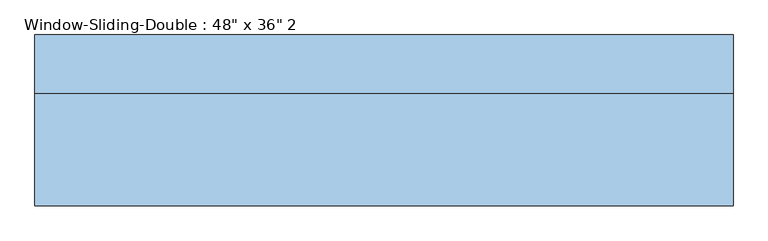
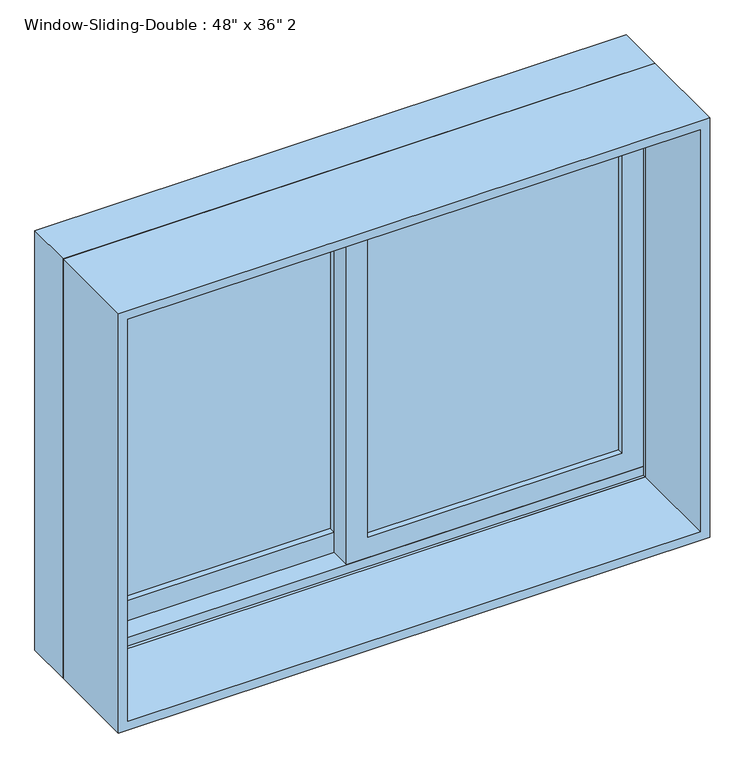
"""IFC4 building model written with IfcOpenShell, lengths in millimetres: window geometry."""

from ifc_helpers import new_model, si_unit, frame, origin, place, context, project, spatial, polyline, outline, extrude, faceted_brep, source, transform, mapped, element, save


def window_d8e423f6(model_context):
    return source(origin(), model_context, "Body", "SolidModel", [
        faceted_brep([(-609.6, 53.34, 914.4), (-609.6, 154.94, 914.4), (609.6, 154.94, 914.4), (609.6, 53.34, 914.4), (-568.6778905, 154.94, 1787.8778905), (-568.6778905, 148.59, 1787.8778905), (-568.6778905, 148.59, 933.45), (-568.6778905, 154.94, 933.45), (568.6778905, 148.59, 1787.8778905), (568.6778905, 148.59, 933.45), (590.55, 148.59, 933.45), (590.55, 148.59, 1809.75), (-590.55, 148.59, 1809.75), (-590.55, 148.59, 933.45), (-590.55, 53.34, 1809.75), (-590.55, 53.34, 933.45), (-590.55, 59.69, 933.45), (-590.55, 59.69, 952.5), (-590.55, 104.14, 952.5), (-590.55, 104.14, 933.45), (609.6, 53.34, 1828.8), (-609.6, 53.34, 1828.8), (590.55, 53.34, 1809.75), (590.55, 53.34, 933.45), (-609.6, 154.94, 1828.8), (609.6, 154.94, 1828.8), (568.6778905, 154.94, 933.45), (568.6778905, 154.94, 1787.8778905), (590.55, 104.14, 933.45), (590.55, 104.14, 952.5), (590.55, 59.69, 952.5), (590.55, 59.69, 933.45)], [[[0, 1, 2, 3]], [[4, 5, 6, 7]], [[5, 8, 9, 10, 11, 12, 13, 6]], [[12, 14, 15, 16, 17, 18, 19, 13]], [[0, 3, 20, 21], [22, 23, 15, 14]], [[24, 1, 0, 21]], [[2, 1, 24, 25], [4, 7, 26, 27]], [[5, 4, 27, 8]], [[12, 11, 22, 14]], [[21, 20, 25, 24]], [[8, 27, 26, 9]], [[22, 11, 10, 28, 29, 30, 31, 23]], [[20, 3, 2, 25]], [[26, 7, 6, 13, 19, 28, 10, 9]], [[28, 19, 18, 29]], [[29, 18, 17, 30]], [[30, 17, 16, 31]], [[15, 23, 31, 16]]]),
        extrude(outline(polyline([(1828.8, -609.6), (914.4, -609.6), (914.4, 609.6), (1828.8, 609.6), (1828.8, -609.6)]), holes=[polyline([(1809.75, 590.55), (933.45, 590.55), (933.45, -590.55), (1809.75, -590.55), (1809.75, 590.55)])]), frame((0.0, -143.51, 0.0), z_axis=(0.0, 1.0, 0.0), x_axis=(0.0, 0.0, 1.0)), (0.0, 0.0, 1.0), 196.85),
        extrude(outline(polyline([(546.1, 91.44), (546.1, 85.09), (22.225, 85.09), (22.225, 91.44), (546.1, 91.44)])), frame((0.0, 0.0, 996.95), z_axis=(0.0, 0.0, 1.0), x_axis=(1.0, 0.0, 0.0)), (0.0, 0.0, 1.0), 768.35),
        extrude(outline(polyline([(546.1, 78.74), (546.1, 72.39), (22.225, 72.39), (22.225, 78.74), (546.1, 78.74)])), frame((0.0, 0.0, 996.95), z_axis=(0.0, 0.0, 1.0), x_axis=(1.0, 0.0, 0.0)), (0.0, 0.0, 1.0), 768.35),
        extrude(outline(polyline([(-22.225, 135.89), (-22.225, 129.54), (-546.1, 129.54), (-546.1, 135.89), (-22.225, 135.89)])), frame((0.0, 0.0, 996.95), z_axis=(0.0, 0.0, 1.0), x_axis=(1.0, 0.0, 0.0)), (0.0, 0.0, 1.0), 768.35),
        extrude(outline(polyline([(-22.225, 123.19), (-22.225, 116.84), (-546.1, 116.84), (-546.1, 123.19), (-22.225, 123.19)])), frame((0.0, 0.0, 996.95), z_axis=(0.0, 0.0, 1.0), x_axis=(1.0, 0.0, 0.0)), (0.0, 0.0, 1.0), 768.35),
        extrude(outline(polyline([(933.45, -590.55), (933.45, 22.225), (1809.75, 22.225), (1809.75, -590.55), (933.45, -590.55)]), holes=[polyline([(1765.3, -22.225), (996.95, -22.225), (996.95, -546.1), (1765.3, -546.1), (1765.3, -22.225)])]), frame((0.0, 104.14, 0.0), z_axis=(0.0, 1.0, 0.0), x_axis=(0.0, 0.0, 1.0)), (0.0, 0.0, 1.0), 44.45),
        extrude(outline(polyline([(952.5, 590.55), (1809.75, 590.55), (1809.75, -22.225), (952.5, -22.225), (952.5, 590.55)]), holes=[polyline([(996.95, 22.225), (1765.3, 22.225), (1765.3, 546.1), (996.95, 546.1), (996.95, 22.225)])]), frame((0.0, 59.69, 0.0), z_axis=(0.0, 1.0, 0.0), x_axis=(0.0, 0.0, 1.0)), (0.0, 0.0, 1.0), 44.45),
    ])


if __name__ == "__main__":
    model = new_model("IFC4")
    model_context = context("Model", 3, world=origin())
    ifc_project = project(units=[si_unit("LENGTHUNIT", "METRE", prefix="MILLI")], contexts=[model_context])
    site = spatial("IfcSite", under=ifc_project)
    building = spatial("IfcBuilding", under=site)
    placement = place(None, origin())
    window_shape = window_d8e423f6(model_context)
    element("IfcWindow", 1, ObjectType="Window-Sliding-Double : 48\" x 36\" 2", at=placement, inside=building, context=model_context, shape_type="MappedRepresentation", body=[
        mapped(window_shape, transform((0.0, 0.0, 0.0), x_axis=(1.0, 0.0, 0.0), y_axis=(0.0, 1.0, 0.0), z_axis=(0.0, 0.0, 1.0))),
    ])
    save(model, "model.ifc")

# Revit data of these elements
# Type "Window-Sliding-Double : 48\" x 36\" 2"
#   Type Mark = "16"
#   Fire Rating = "0.5h"
#   Assembly Code = "B2020100"
#   Analytic Construction = "Double glazing - domestic"
#   Window Inset [instance default] = 0' - 0"
#   Wall Thickness [instance default] = 0' - 6"
#   Visual Light Transmittance = 0.81
#   Thermal Resistance (R) = 0.319569 (m²·K)/W
#   Solar Heat Gain Coefficient = 0.76
#   Muntin Width = 1' - 8 5/8"
#   Muntin Height = 2' - 6 1/4"
#   Interior Wall Closure [instance default] = 0' - 2 3/4"
#   Heat Transfer Coefficient (U) = 3.12929 W/(m²·K)
#   Frame Extension [instance default] = 0' - 0 1/4"
#   Exterior Wall Closure [instance default] = 0' - 1 1/4"
#   Rough Width = 4' - 0 1/2"
#   Rough Height = 3' - 0 1/2"
#   Height = 3' - 0"
#   Extension Jamb [instance default] = 0' - 2 3/4"
#   Default Sill Height = 3' - 0"
#   Width = 4' - 0"
#   Interior Trim Visibility [instance default] = yes
#   Indicator Visibility [instance default] = yes
#   Exterior Trim Visibility [instance default] = yes
#   Muntin Visibility = no
#   Extension Jamb Visibility [instance default] = yes
#   Muntin Pattern = Muntin Pattern_2x2 : Muntin Pattern_2x2
#   Interior Trim Material = accent 2
#   Interior Trim = Trim-Window-Interior-Flat : Picture Frame
#   Interior Frame Material = accent 2
#   Glass Panel Material = Glass
#   Exterior Trim Material = accent 2
#   Exterior Trim = Trim-Window-Exterior-Flat : with Sill
#   Exterior Frame Material = accent 2
#   Wall Closure = (empty or 0)
# Element 1 (IfcWindow, "Window-Sliding-Double : 48\" x 36\" 2")
#   Wall Thickness = 0' - 11"
#   Extension Jamb = 0' - 7 3/4"
#   Materials on its faces: "accent 2", "Glass"
# Materials
#   "accent 2": class "Wood", colour RGB 80 80 80, transparency 0, Description = "Wood framing, thermal airspace", Cost = 0
#   "Glass": class "Glass", colour RGB 236 240 239, transparency 0.85, Description = "Soda Lime Glass", Cost = 0
